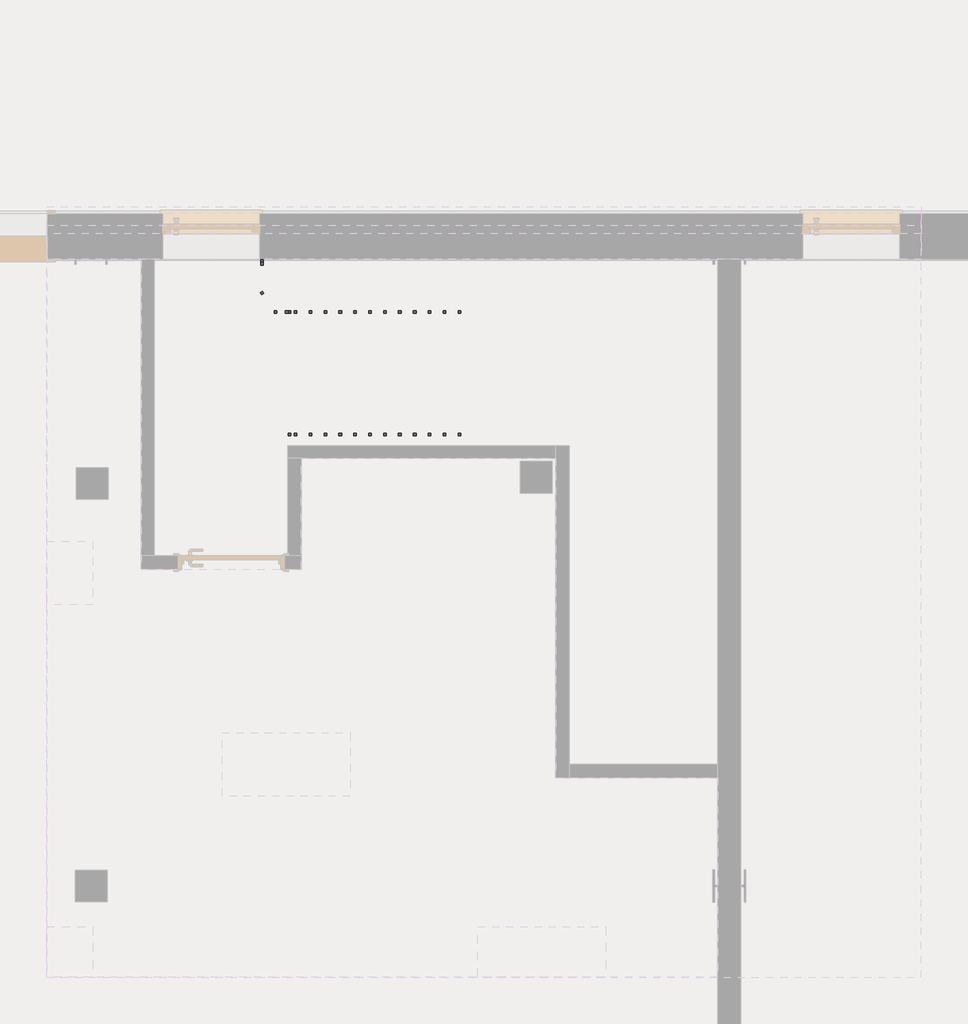
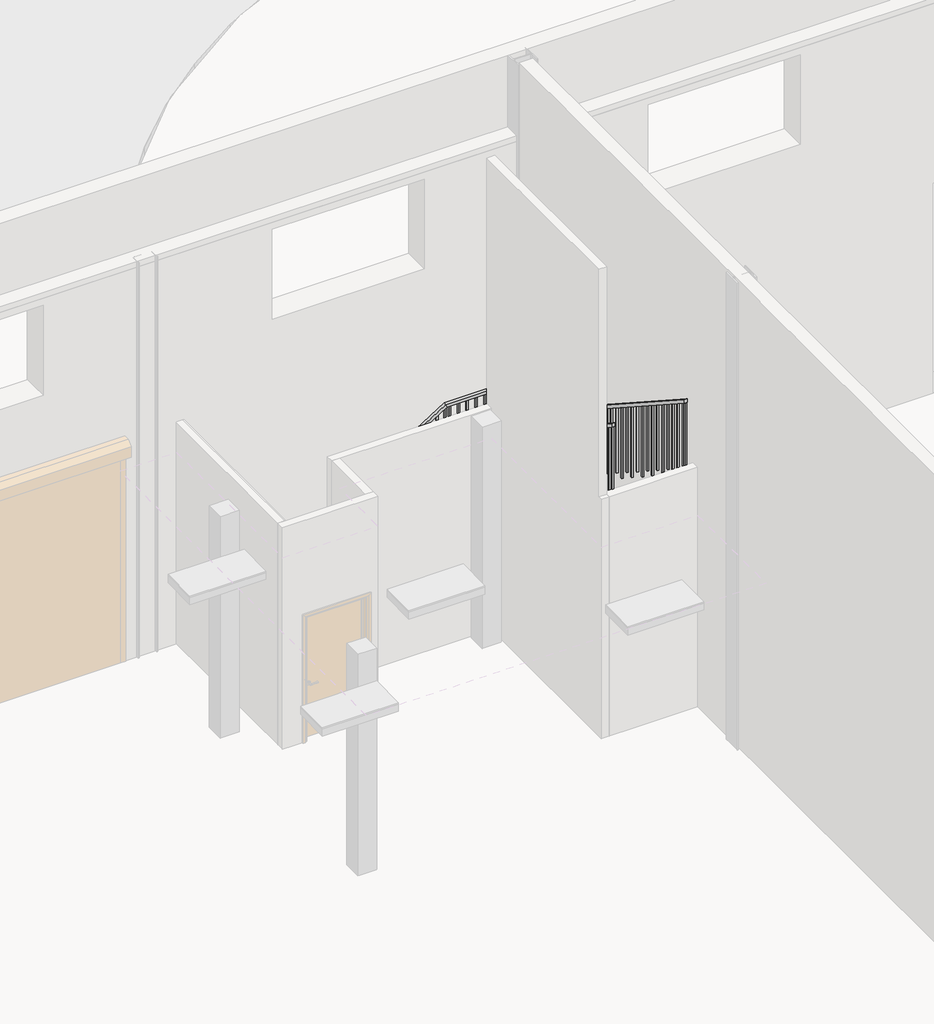
# One storey, part 10 of 13: 3 railings.
"""IFC4 building model written with IfcOpenShell, lengths in millimetres."""

from ifc_helpers import new_model, si_unit, frame, origin, place, context, project, spatial, polyline, outline, extrude, faceted_brep, element, save

model = new_model("IFC4")

# Units and contexts
model_context = context("Model", 3, world=origin())
ifc_project = project(units=[si_unit("LENGTHUNIT", "METRE", prefix="MILLI")], contexts=[model_context])

# Site, building, storey
site = spatial("IfcSite", under=ifc_project)
building = spatial("IfcBuilding", under=site)
storey = spatial("IfcBuildingStorey", under=building, Name="L0 - Ground Floor (Shadows On)", Elevation=0.0)

# Railings
placement = place(None, origin())
element("IfcRailing", 1, ObjectType="1100mm", at=placement, inside=storey, context=model_context, shape_type="SolidModel", body=[
    faceted_brep([(6712.9446543, 5212.4222729, 1286.5612648), (6712.9446543, 5212.4222729, 1227.4016553), (6712.9446543, 5162.4222729, 1227.4016553), (6712.9446543, 5162.4222729, 1286.5612648), (9292.9446543, 5212.4222729, 2918.1818182), (9307.4282868, 5212.4222729, 2868.1818182), (9307.4282868, 5162.4222729, 2868.1818182), (9292.9446543, 5162.4222729, 2918.1818182), (9390.9278057, 5212.4222729, 2918.1818182), (9440.9278057, 5212.4222729, 2868.1818182), (9440.9278057, 5162.4222729, 2868.1818182), (9390.9278057, 5162.4222729, 2918.1818182), (9390.9278057, 5212.4222729, 3148.4415584), (9440.9278057, 5212.4222729, 3098.4415584), (9440.9278057, 5162.4222729, 3098.4415584), (9390.9278057, 5162.4222729, 3148.4415584), (9515.9278057, 5212.4222729, 3148.4415584), (9515.9278057, 5212.4222729, 3098.4415584), (9465.9278057, 5162.4222729, 3098.4415584), (9465.9278057, 5162.4222729, 3148.4415584), (9515.9278057, 5087.4222729, 3148.4415584), (9515.9278057, 5072.6126873, 3098.4415584), (9465.9278057, 5072.6126873, 3098.4415584), (9465.9278057, 5087.4222729, 3148.4415584), (9515.9278057, 2082.0222729, 5100.0), (9465.9278057, 2082.0222729, 5100.0), (9465.9278057, 2082.0222729, 5040.383386), (9515.9278057, 2082.0222729, 5040.383386)], [[[0, 1, 2, 3]], [[1, 0, 4, 5]], [[2, 1, 5, 6]], [[3, 2, 6, 7]], [[0, 3, 7, 4]], [[5, 4, 8, 9]], [[6, 5, 9, 10]], [[7, 6, 10, 11]], [[4, 7, 11, 8]], [[9, 8, 12, 13]], [[10, 9, 13, 14]], [[11, 10, 14, 15]], [[8, 11, 15, 12]], [[13, 12, 16, 17]], [[14, 13, 17, 18]], [[15, 14, 18, 19]], [[12, 15, 19, 16]], [[17, 16, 20, 21]], [[18, 17, 21, 22]], [[19, 18, 22, 23]], [[16, 19, 23, 20]], [[24, 25, 26, 27]], [[21, 20, 24, 27]], [[22, 21, 27, 26]], [[23, 22, 26, 25]], [[20, 23, 25, 24]]]),
    extrude(outline(polyline([(2189.9222729, 4970.3184509), (2189.9222729, 3818.1818182), (2164.9222729, 3818.1818182), (2164.9222729, 4986.5522172), (2189.9222729, 4970.3184509)])), frame((9478.4278057, 0.0, 0.0), z_axis=(1.0, 0.0, 0.0), x_axis=(0.0, 1.0, 0.0)), (0.0, 0.0, 1.0), 25.0),
    extrude(outline(polyline([(2329.9222729, 4879.40936), (2329.9222729, 3818.1818182), (2304.9222729, 3818.1818182), (2304.9222729, 4895.6431263), (2329.9222729, 4879.40936)])), frame((9478.4278057, 0.0, 0.0), z_axis=(1.0, 0.0, 0.0), x_axis=(0.0, 1.0, 0.0)), (0.0, 0.0, 1.0), 25.0),
    extrude(outline(polyline([(2469.9222729, 4788.5002691), (2469.9222729, 3636.3636364), (2444.9222729, 3636.3636364), (2444.9222729, 4804.7340354), (2469.9222729, 4788.5002691)])), frame((9478.4278057, 0.0, 0.0), z_axis=(1.0, 0.0, 0.0), x_axis=(0.0, 1.0, 0.0)), (0.0, 0.0, 1.0), 25.0),
    extrude(outline(polyline([(2609.9222729, 4697.5911782), (2609.9222729, 3636.3636364), (2584.9222729, 3636.3636364), (2584.9222729, 4713.8249444), (2609.9222729, 4697.5911782)])), frame((9478.4278057, 0.0, 0.0), z_axis=(1.0, 0.0, 0.0), x_axis=(0.0, 1.0, 0.0)), (0.0, 0.0, 1.0), 25.0),
    extrude(outline(polyline([(2749.9222729, 4606.6820873), (2749.9222729, 3454.5454545), (2724.9222729, 3454.5454545), (2724.9222729, 4622.9158535), (2749.9222729, 4606.6820873)])), frame((9478.4278057, 0.0, 0.0), z_axis=(1.0, 0.0, 0.0), x_axis=(0.0, 1.0, 0.0)), (0.0, 0.0, 1.0), 25.0),
    extrude(outline(polyline([(2889.9222729, 4515.7729964), (2889.9222729, 3454.5454545), (2864.9222729, 3454.5454545), (2864.9222729, 4532.0067626), (2889.9222729, 4515.7729964)])), frame((9478.4278057, 0.0, 0.0), z_axis=(1.0, 0.0, 0.0), x_axis=(0.0, 1.0, 0.0)), (0.0, 0.0, 1.0), 25.0),
    extrude(outline(polyline([(3029.9222729, 4424.8639055), (3029.9222729, 3272.7272727), (3004.9222729, 3272.7272727), (3004.9222729, 4441.0976717), (3029.9222729, 4424.8639055)])), frame((9478.4278057, 0.0, 0.0), z_axis=(1.0, 0.0, 0.0), x_axis=(0.0, 1.0, 0.0)), (0.0, 0.0, 1.0), 25.0),
    extrude(outline(polyline([(3169.9222729, 4333.9548146), (3169.9222729, 3272.7272727), (3144.9222729, 3272.7272727), (3144.9222729, 4350.1885808), (3169.9222729, 4333.9548146)])), frame((9478.4278057, 0.0, 0.0), z_axis=(1.0, 0.0, 0.0), x_axis=(0.0, 1.0, 0.0)), (0.0, 0.0, 1.0), 25.0),
    extrude(outline(polyline([(3309.9222729, 4243.0457237), (3309.9222729, 3090.9090909), (3284.9222729, 3090.9090909), (3284.9222729, 4259.2794899), (3309.9222729, 4243.0457237)])), frame((9478.4278057, 0.0, 0.0), z_axis=(1.0, 0.0, 0.0), x_axis=(0.0, 1.0, 0.0)), (0.0, 0.0, 1.0), 25.0),
    extrude(outline(polyline([(3449.9222729, 4152.1366328), (3449.9222729, 3090.9090909), (3424.9222729, 3090.9090909), (3424.9222729, 4168.370399), (3449.9222729, 4152.1366328)])), frame((9478.4278057, 0.0, 0.0), z_axis=(1.0, 0.0, 0.0), x_axis=(0.0, 1.0, 0.0)), (0.0, 0.0, 1.0), 25.0),
    extrude(outline(polyline([(3589.9222729, 4061.2275418), (3589.9222729, 2909.0909091), (3564.9222729, 2909.0909091), (3564.9222729, 4077.4613081), (3589.9222729, 4061.2275418)])), frame((9478.4278057, 0.0, 0.0), z_axis=(1.0, 0.0, 0.0), x_axis=(0.0, 1.0, 0.0)), (0.0, 0.0, 1.0), 25.0),
    extrude(outline(polyline([(3729.9222729, 3970.3184509), (3729.9222729, 2909.0909091), (3704.9222729, 2909.0909091), (3704.9222729, 3986.5522172), (3729.9222729, 3970.3184509)])), frame((9478.4278057, 0.0, 0.0), z_axis=(1.0, 0.0, 0.0), x_axis=(0.0, 1.0, 0.0)), (0.0, 0.0, 1.0), 25.0),
    extrude(outline(polyline([(3869.9222729, 3879.40936), (3869.9222729, 2727.2727273), (3844.9222729, 2727.2727273), (3844.9222729, 3895.6431263), (3869.9222729, 3879.40936)])), frame((9478.4278057, 0.0, 0.0), z_axis=(1.0, 0.0, 0.0), x_axis=(0.0, 1.0, 0.0)), (0.0, 0.0, 1.0), 25.0),
    extrude(outline(polyline([(4009.9222729, 3788.5002691), (4009.9222729, 2727.2727273), (3984.9222729, 2727.2727273), (3984.9222729, 3804.7340354), (4009.9222729, 3788.5002691)])), frame((9478.4278057, 0.0, 0.0), z_axis=(1.0, 0.0, 0.0), x_axis=(0.0, 1.0, 0.0)), (0.0, 0.0, 1.0), 25.0),
    extrude(outline(polyline([(4149.9222729, 3697.5911782), (4149.9222729, 2545.4545455), (4124.9222729, 2545.4545455), (4124.9222729, 3713.8249444), (4149.9222729, 3697.5911782)])), frame((9478.4278057, 0.0, 0.0), z_axis=(1.0, 0.0, 0.0), x_axis=(0.0, 1.0, 0.0)), (0.0, 0.0, 1.0), 25.0),
    extrude(outline(polyline([(4289.9222729, 3606.6820873), (4289.9222729, 2545.4545455), (4264.9222729, 2545.4545455), (4264.9222729, 3622.9158535), (4289.9222729, 3606.6820873)])), frame((9478.4278057, 0.0, 0.0), z_axis=(1.0, 0.0, 0.0), x_axis=(0.0, 1.0, 0.0)), (0.0, 0.0, 1.0), 25.0),
    extrude(outline(polyline([(4429.9222729, 3515.7729964), (4429.9222729, 2363.6363636), (4404.9222729, 2363.6363636), (4404.9222729, 3532.0067626), (4429.9222729, 3515.7729964)])), frame((9478.4278057, 0.0, 0.0), z_axis=(1.0, 0.0, 0.0), x_axis=(0.0, 1.0, 0.0)), (0.0, 0.0, 1.0), 25.0),
    extrude(outline(polyline([(4569.9222729, 3424.8639055), (4569.9222729, 2363.6363636), (4544.9222729, 2363.6363636), (4544.9222729, 3441.0976717), (4569.9222729, 3424.8639055)])), frame((9478.4278057, 0.0, 0.0), z_axis=(1.0, 0.0, 0.0), x_axis=(0.0, 1.0, 0.0)), (0.0, 0.0, 1.0), 25.0),
    extrude(outline(polyline([(4709.9222729, 3333.9548146), (4709.9222729, 2181.8181818), (4684.9222729, 2181.8181818), (4684.9222729, 3350.1885808), (4709.9222729, 3333.9548146)])), frame((9478.4278057, 0.0, 0.0), z_axis=(1.0, 0.0, 0.0), x_axis=(0.0, 1.0, 0.0)), (0.0, 0.0, 1.0), 25.0),
    extrude(outline(polyline([(4849.9222729, 3243.0457237), (4849.9222729, 2181.8181818), (4824.9222729, 2181.8181818), (4824.9222729, 3259.2794899), (4849.9222729, 3243.0457237)])), frame((9478.4278057, 0.0, 0.0), z_axis=(1.0, 0.0, 0.0), x_axis=(0.0, 1.0, 0.0)), (0.0, 0.0, 1.0), 25.0),
    extrude(outline(polyline([(4989.9222729, 3152.1366328), (4989.9222729, 2000.0), (4964.9222729, 2000.0), (4964.9222729, 3168.370399), (4989.9222729, 3152.1366328)])), frame((9478.4278057, 0.0, 0.0), z_axis=(1.0, 0.0, 0.0), x_axis=(0.0, 1.0, 0.0)), (0.0, 0.0, 1.0), 25.0),
    extrude(outline(polyline([(9478.4278057, 5129.9222729), (9503.4278057, 5129.9222729), (9503.4278057, 5104.9222729), (9478.4278057, 5104.9222729), (9478.4278057, 5129.9222729)])), frame((0.0, 0.0, 2000.0), z_axis=(0.0, 0.0, 1.0), x_axis=(1.0, 0.0, 0.0)), (0.0, 0.0, 1.0), 1098.4415584),
    extrude(outline(polyline([(9350.4446543, 5174.9222729), (9350.4446543, 5199.9222729), (9375.4446543, 5199.9222729), (9375.4446543, 5174.9222729), (9350.4446543, 5174.9222729)])), frame((0.0, 0.0, 1818.1818182), z_axis=(0.0, 0.0, 1.0), x_axis=(1.0, 0.0, 0.0)), (0.0, 0.0, 1.0), 1050.0),
    extrude(outline(polyline([(2768.9036316, 9150.4446543), (1636.3636364, 9150.4446543), (1636.3636364, 9175.4446543), (2784.7139083, 9175.4446543), (2768.9036316, 9150.4446543)])), frame((0.0, 5174.9222729, 0.0), z_axis=(0.0, 1.0, 0.0), x_axis=(0.0, 0.0, 1.0)), (0.0, 0.0, 1.0), 25.0),
    extrude(outline(polyline([(2680.3660822, 9010.4446543), (1636.3636364, 9010.4446543), (1636.3636364, 9035.4446543), (2696.1763589, 9035.4446543), (2680.3660822, 9010.4446543)])), frame((0.0, 5174.9222729, 0.0), z_axis=(0.0, 1.0, 0.0), x_axis=(0.0, 0.0, 1.0)), (0.0, 0.0, 1.0), 25.0),
    extrude(outline(polyline([(2591.8285328, 8870.4446543), (1454.5454545, 8870.4446543), (1454.5454545, 8895.4446543), (2607.6388095, 8895.4446543), (2591.8285328, 8870.4446543)])), frame((0.0, 5174.9222729, 0.0), z_axis=(0.0, 1.0, 0.0), x_axis=(0.0, 0.0, 1.0)), (0.0, 0.0, 1.0), 25.0),
    extrude(outline(polyline([(2503.2909834, 8730.4446543), (1454.5454545, 8730.4446543), (1454.5454545, 8755.4446543), (2519.1012601, 8755.4446543), (2503.2909834, 8730.4446543)])), frame((0.0, 5174.9222729, 0.0), z_axis=(0.0, 1.0, 0.0), x_axis=(0.0, 0.0, 1.0)), (0.0, 0.0, 1.0), 25.0),
    extrude(outline(polyline([(2414.753434, 8590.4446543), (1272.7272727, 8590.4446543), (1272.7272727, 8615.4446543), (2430.5637107, 8615.4446543), (2414.753434, 8590.4446543)])), frame((0.0, 5174.9222729, 0.0), z_axis=(0.0, 1.0, 0.0), x_axis=(0.0, 0.0, 1.0)), (0.0, 0.0, 1.0), 25.0),
    extrude(outline(polyline([(2326.2158846, 8450.4446543), (1272.7272727, 8450.4446543), (1272.7272727, 8475.4446543), (2342.0261613, 8475.4446543), (2326.2158846, 8450.4446543)])), frame((0.0, 5174.9222729, 0.0), z_axis=(0.0, 1.0, 0.0), x_axis=(0.0, 0.0, 1.0)), (0.0, 0.0, 1.0), 25.0),
    extrude(outline(polyline([(2237.6783352, 8310.4446543), (1090.9090909, 8310.4446543), (1090.9090909, 8335.4446543), (2253.4886119, 8335.4446543), (2237.6783352, 8310.4446543)])), frame((0.0, 5174.9222729, 0.0), z_axis=(0.0, 1.0, 0.0), x_axis=(0.0, 0.0, 1.0)), (0.0, 0.0, 1.0), 25.0),
    extrude(outline(polyline([(2149.1407858, 8170.4446543), (1090.9090909, 8170.4446543), (1090.9090909, 8195.4446543), (2164.9510624, 8195.4446543), (2149.1407858, 8170.4446543)])), frame((0.0, 5174.9222729, 0.0), z_axis=(0.0, 1.0, 0.0), x_axis=(0.0, 0.0, 1.0)), (0.0, 0.0, 1.0), 25.0),
    extrude(outline(polyline([(2060.6032364, 8030.4446543), (909.0909091, 8030.4446543), (909.0909091, 8055.4446543), (2076.413513, 8055.4446543), (2060.6032364, 8030.4446543)])), frame((0.0, 5174.9222729, 0.0), z_axis=(0.0, 1.0, 0.0), x_axis=(0.0, 0.0, 1.0)), (0.0, 0.0, 1.0), 25.0),
    extrude(outline(polyline([(1972.065687, 7890.4446543), (909.0909091, 7890.4446543), (909.0909091, 7915.4446543), (1987.8759636, 7915.4446543), (1972.065687, 7890.4446543)])), frame((0.0, 5174.9222729, 0.0), z_axis=(0.0, 1.0, 0.0), x_axis=(0.0, 0.0, 1.0)), (0.0, 0.0, 1.0), 25.0),
    extrude(outline(polyline([(1883.5281375, 7750.4446543), (727.2727273, 7750.4446543), (727.2727273, 7775.4446543), (1899.3384142, 7775.4446543), (1883.5281375, 7750.4446543)])), frame((0.0, 5174.9222729, 0.0), z_axis=(0.0, 1.0, 0.0), x_axis=(0.0, 0.0, 1.0)), (0.0, 0.0, 1.0), 25.0),
    extrude(outline(polyline([(1794.9905881, 7610.4446543), (727.2727273, 7610.4446543), (727.2727273, 7635.4446543), (1810.8008648, 7635.4446543), (1794.9905881, 7610.4446543)])), frame((0.0, 5174.9222729, 0.0), z_axis=(0.0, 1.0, 0.0), x_axis=(0.0, 0.0, 1.0)), (0.0, 0.0, 1.0), 25.0),
    extrude(outline(polyline([(1706.4530387, 7470.4446543), (545.4545455, 7470.4446543), (545.4545455, 7495.4446543), (1722.2633154, 7495.4446543), (1706.4530387, 7470.4446543)])), frame((0.0, 5174.9222729, 0.0), z_axis=(0.0, 1.0, 0.0), x_axis=(0.0, 0.0, 1.0)), (0.0, 0.0, 1.0), 25.0),
    extrude(outline(polyline([(1617.9154893, 7330.4446543), (545.4545455, 7330.4446543), (545.4545455, 7355.4446543), (1633.725766, 7355.4446543), (1617.9154893, 7330.4446543)])), frame((0.0, 5174.9222729, 0.0), z_axis=(0.0, 1.0, 0.0), x_axis=(0.0, 0.0, 1.0)), (0.0, 0.0, 1.0), 25.0),
    extrude(outline(polyline([(1529.3779399, 7190.4446543), (363.6363636, 7190.4446543), (363.6363636, 7215.4446543), (1545.1882166, 7215.4446543), (1529.3779399, 7190.4446543)])), frame((0.0, 5174.9222729, 0.0), z_axis=(0.0, 1.0, 0.0), x_axis=(0.0, 0.0, 1.0)), (0.0, 0.0, 1.0), 25.0),
    extrude(outline(polyline([(1440.8403905, 7050.4446543), (363.6363636, 7050.4446543), (363.6363636, 7075.4446543), (1456.6506672, 7075.4446543), (1440.8403905, 7050.4446543)])), frame((0.0, 5174.9222729, 0.0), z_axis=(0.0, 1.0, 0.0), x_axis=(0.0, 0.0, 1.0)), (0.0, 0.0, 1.0), 25.0),
    extrude(outline(polyline([(1352.3028411, 6910.4446543), (181.8181818, 6910.4446543), (181.8181818, 6935.4446543), (1368.1131178, 6935.4446543), (1352.3028411, 6910.4446543)])), frame((0.0, 5174.9222729, 0.0), z_axis=(0.0, 1.0, 0.0), x_axis=(0.0, 0.0, 1.0)), (0.0, 0.0, 1.0), 25.0),
    extrude(outline(polyline([(1263.7652917, 6770.4446543), (181.8181818, 6770.4446543), (181.8181818, 6795.4446543), (1279.5755684, 6795.4446543), (1263.7652917, 6770.4446543)])), frame((0.0, 5174.9222729, 0.0), z_axis=(0.0, 1.0, 0.0), x_axis=(0.0, 0.0, 1.0)), (0.0, 0.0, 1.0), 25.0),
    extrude(outline(polyline([(9478.4278057, 5199.9222729), (9503.4278057, 5199.9222729), (9503.4278057, 5174.9222729), (9478.4278057, 5174.9222729), (9478.4278057, 5199.9222729)])), frame((0.0, 0.0, 1818.1818182), z_axis=(0.0, 0.0, 1.0), x_axis=(1.0, 0.0, 0.0)), (0.0, 0.0, 1.0), 1280.2597403),
    extrude(outline(polyline([(2851.1170704, 9280.4446543), (1818.1818182, 9280.4446543), (1818.1818182, 9305.4446543), (2866.927347, 9305.4446543), (2851.1170704, 9280.4446543)])), frame((0.0, 5174.9222729, 0.0), z_axis=(0.0, 1.0, 0.0), x_axis=(0.0, 0.0, 1.0)), (0.0, 0.0, 1.0), 25.0),
    extrude(outline(polyline([(2107.0222729, 5024.1496198), (2107.0222729, 3818.1818182), (2082.0222729, 3818.1818182), (2082.0222729, 5040.383386), (2107.0222729, 5024.1496198)])), frame((9478.4278057, 0.0, 0.0), z_axis=(1.0, 0.0, 0.0), x_axis=(0.0, 1.0, 0.0)), (0.0, 0.0, 1.0), 25.0),
    extrude(outline(polyline([(1227.4016553, 6712.9446543), (181.8181818, 6712.9446543), (181.8181818, 6737.9446543), (1243.211932, 6737.9446543), (1227.4016553, 6712.9446543)])), frame((0.0, 5174.9222729, 0.0), z_axis=(0.0, 1.0, 0.0), x_axis=(0.0, 0.0, 1.0)), (0.0, 0.0, 1.0), 25.0),
])
element("IfcRailing", 2, ObjectType="1100mm", at=placement, inside=storey, context=model_context, shape_type="SolidModel", body=[
    faceted_brep([(6712.9446543, 6361.6222729, 1286.5612648), (6712.9446543, 6361.6222729, 1227.4016553), (6712.9446543, 6311.6222729, 1227.4016553), (6712.9446543, 6311.6222729, 1286.5612648), (9292.9446543, 6361.6222729, 2918.1818182), (9307.4282868, 6361.6222729, 2868.1818182), (9307.4282868, 6311.6222729, 2868.1818182), (9292.9446543, 6311.6222729, 2918.1818182), (10665.1278057, 6361.6222729, 2918.1818182), (10665.1278057, 6361.6222729, 2868.1818182), (10615.1278057, 6311.6222729, 2868.1818182), (10615.1278057, 6311.6222729, 2918.1818182), (10665.1278057, 5442.0222729, 2918.1818182), (10665.1278057, 5427.2126873, 2868.1818182), (10615.1278057, 5427.2126873, 2868.1818182), (10615.1278057, 5442.0222729, 2918.1818182), (10665.1278057, 2082.0222729, 5100.0), (10615.1278057, 2082.0222729, 5100.0), (10615.1278057, 2082.0222729, 5040.383386), (10665.1278057, 2082.0222729, 5040.383386)], [[[0, 1, 2, 3]], [[1, 0, 4, 5]], [[2, 1, 5, 6]], [[3, 2, 6, 7]], [[0, 3, 7, 4]], [[5, 4, 8, 9]], [[6, 5, 9, 10]], [[7, 6, 10, 11]], [[4, 7, 11, 8]], [[9, 8, 12, 13]], [[10, 9, 13, 14]], [[11, 10, 14, 15]], [[8, 11, 15, 12]], [[16, 17, 18, 19]], [[13, 12, 16, 19]], [[14, 13, 19, 18]], [[15, 14, 18, 17]], [[12, 15, 17, 16]]]),
    extrude(outline(polyline([(2164.5222729, 3818.1818182), (2139.5222729, 3818.1818182), (2139.5222729, 5003.0457237), (2164.5222729, 4986.8119574), (2164.5222729, 3818.1818182)])), frame((10627.6278057, 0.0, 0.0), z_axis=(1.0, 0.0, 0.0), x_axis=(0.0, 1.0, 0.0)), (0.0, 0.0, 1.0), 25.0),
    extrude(outline(polyline([(2304.5222729, 3818.1818182), (2279.5222729, 3818.1818182), (2279.5222729, 4912.1366328), (2304.5222729, 4895.9028665), (2304.5222729, 3818.1818182)])), frame((10627.6278057, 0.0, 0.0), z_axis=(1.0, 0.0, 0.0), x_axis=(0.0, 1.0, 0.0)), (0.0, 0.0, 1.0), 25.0),
    extrude(outline(polyline([(2444.5222729, 3636.3636364), (2419.5222729, 3636.3636364), (2419.5222729, 4821.2275418), (2444.5222729, 4804.9937756), (2444.5222729, 3636.3636364)])), frame((10627.6278057, 0.0, 0.0), z_axis=(1.0, 0.0, 0.0), x_axis=(0.0, 1.0, 0.0)), (0.0, 0.0, 1.0), 25.0),
    extrude(outline(polyline([(2584.5222729, 3636.3636364), (2559.5222729, 3636.3636364), (2559.5222729, 4730.3184509), (2584.5222729, 4714.0846847), (2584.5222729, 3636.3636364)])), frame((10627.6278057, 0.0, 0.0), z_axis=(1.0, 0.0, 0.0), x_axis=(0.0, 1.0, 0.0)), (0.0, 0.0, 1.0), 25.0),
    extrude(outline(polyline([(2724.5222729, 3454.5454545), (2699.5222729, 3454.5454545), (2699.5222729, 4639.40936), (2724.5222729, 4623.1755938), (2724.5222729, 3454.5454545)])), frame((10627.6278057, 0.0, 0.0), z_axis=(1.0, 0.0, 0.0), x_axis=(0.0, 1.0, 0.0)), (0.0, 0.0, 1.0), 25.0),
    extrude(outline(polyline([(2864.5222729, 3454.5454545), (2839.5222729, 3454.5454545), (2839.5222729, 4548.5002691), (2864.5222729, 4532.2665029), (2864.5222729, 3454.5454545)])), frame((10627.6278057, 0.0, 0.0), z_axis=(1.0, 0.0, 0.0), x_axis=(0.0, 1.0, 0.0)), (0.0, 0.0, 1.0), 25.0),
    extrude(outline(polyline([(3004.5222729, 3272.7272727), (2979.5222729, 3272.7272727), (2979.5222729, 4457.5911782), (3004.5222729, 4441.357412), (3004.5222729, 3272.7272727)])), frame((10627.6278057, 0.0, 0.0), z_axis=(1.0, 0.0, 0.0), x_axis=(0.0, 1.0, 0.0)), (0.0, 0.0, 1.0), 25.0),
    extrude(outline(polyline([(3144.5222729, 3272.7272727), (3119.5222729, 3272.7272727), (3119.5222729, 4366.6820873), (3144.5222729, 4350.4483211), (3144.5222729, 3272.7272727)])), frame((10627.6278057, 0.0, 0.0), z_axis=(1.0, 0.0, 0.0), x_axis=(0.0, 1.0, 0.0)), (0.0, 0.0, 1.0), 25.0),
    extrude(outline(polyline([(3284.5222729, 3090.9090909), (3259.5222729, 3090.9090909), (3259.5222729, 4275.7729964), (3284.5222729, 4259.5392302), (3284.5222729, 3090.9090909)])), frame((10627.6278057, 0.0, 0.0), z_axis=(1.0, 0.0, 0.0), x_axis=(0.0, 1.0, 0.0)), (0.0, 0.0, 1.0), 25.0),
    extrude(outline(polyline([(3424.5222729, 3090.9090909), (3399.5222729, 3090.9090909), (3399.5222729, 4184.8639055), (3424.5222729, 4168.6301392), (3424.5222729, 3090.9090909)])), frame((10627.6278057, 0.0, 0.0), z_axis=(1.0, 0.0, 0.0), x_axis=(0.0, 1.0, 0.0)), (0.0, 0.0, 1.0), 25.0),
    extrude(outline(polyline([(3564.5222729, 2909.0909091), (3539.5222729, 2909.0909091), (3539.5222729, 4093.9548146), (3564.5222729, 4077.7210483), (3564.5222729, 2909.0909091)])), frame((10627.6278057, 0.0, 0.0), z_axis=(1.0, 0.0, 0.0), x_axis=(0.0, 1.0, 0.0)), (0.0, 0.0, 1.0), 25.0),
    extrude(outline(polyline([(3704.5222729, 2909.0909091), (3679.5222729, 2909.0909091), (3679.5222729, 4003.0457237), (3704.5222729, 3986.8119574), (3704.5222729, 2909.0909091)])), frame((10627.6278057, 0.0, 0.0), z_axis=(1.0, 0.0, 0.0), x_axis=(0.0, 1.0, 0.0)), (0.0, 0.0, 1.0), 25.0),
    extrude(outline(polyline([(3844.5222729, 2727.2727273), (3819.5222729, 2727.2727273), (3819.5222729, 3912.1366328), (3844.5222729, 3895.9028665), (3844.5222729, 2727.2727273)])), frame((10627.6278057, 0.0, 0.0), z_axis=(1.0, 0.0, 0.0), x_axis=(0.0, 1.0, 0.0)), (0.0, 0.0, 1.0), 25.0),
    extrude(outline(polyline([(3984.5222729, 2727.2727273), (3959.5222729, 2727.2727273), (3959.5222729, 3821.2275418), (3984.5222729, 3804.9937756), (3984.5222729, 2727.2727273)])), frame((10627.6278057, 0.0, 0.0), z_axis=(1.0, 0.0, 0.0), x_axis=(0.0, 1.0, 0.0)), (0.0, 0.0, 1.0), 25.0),
    extrude(outline(polyline([(4124.5222729, 2545.4545455), (4099.5222729, 2545.4545455), (4099.5222729, 3730.3184509), (4124.5222729, 3714.0846847), (4124.5222729, 2545.4545455)])), frame((10627.6278057, 0.0, 0.0), z_axis=(1.0, 0.0, 0.0), x_axis=(0.0, 1.0, 0.0)), (0.0, 0.0, 1.0), 25.0),
    extrude(outline(polyline([(4264.5222729, 2545.4545455), (4239.5222729, 2545.4545455), (4239.5222729, 3639.40936), (4264.5222729, 3623.1755938), (4264.5222729, 2545.4545455)])), frame((10627.6278057, 0.0, 0.0), z_axis=(1.0, 0.0, 0.0), x_axis=(0.0, 1.0, 0.0)), (0.0, 0.0, 1.0), 25.0),
    extrude(outline(polyline([(4404.5222729, 2363.6363636), (4379.5222729, 2363.6363636), (4379.5222729, 3548.5002691), (4404.5222729, 3532.2665029), (4404.5222729, 2363.6363636)])), frame((10627.6278057, 0.0, 0.0), z_axis=(1.0, 0.0, 0.0), x_axis=(0.0, 1.0, 0.0)), (0.0, 0.0, 1.0), 25.0),
    extrude(outline(polyline([(4544.5222729, 2363.6363636), (4519.5222729, 2363.6363636), (4519.5222729, 3457.5911782), (4544.5222729, 3441.357412), (4544.5222729, 2363.6363636)])), frame((10627.6278057, 0.0, 0.0), z_axis=(1.0, 0.0, 0.0), x_axis=(0.0, 1.0, 0.0)), (0.0, 0.0, 1.0), 25.0),
    extrude(outline(polyline([(4684.5222729, 2181.8181818), (4659.5222729, 2181.8181818), (4659.5222729, 3366.6820873), (4684.5222729, 3350.4483211), (4684.5222729, 2181.8181818)])), frame((10627.6278057, 0.0, 0.0), z_axis=(1.0, 0.0, 0.0), x_axis=(0.0, 1.0, 0.0)), (0.0, 0.0, 1.0), 25.0),
    extrude(outline(polyline([(4824.5222729, 2181.8181818), (4799.5222729, 2181.8181818), (4799.5222729, 3275.7729964), (4824.5222729, 3259.5392302), (4824.5222729, 2181.8181818)])), frame((10627.6278057, 0.0, 0.0), z_axis=(1.0, 0.0, 0.0), x_axis=(0.0, 1.0, 0.0)), (0.0, 0.0, 1.0), 25.0),
    extrude(outline(polyline([(4964.5222729, 2000.0), (4939.5222729, 2000.0), (4939.5222729, 3184.8639055), (4964.5222729, 3168.6301392), (4964.5222729, 2000.0)])), frame((10627.6278057, 0.0, 0.0), z_axis=(1.0, 0.0, 0.0), x_axis=(0.0, 1.0, 0.0)), (0.0, 0.0, 1.0), 25.0),
    extrude(outline(polyline([(5104.5222729, 2000.0), (5079.5222729, 2000.0), (5079.5222729, 3093.9548146), (5104.5222729, 3077.7210483), (5104.5222729, 2000.0)])), frame((10627.6278057, 0.0, 0.0), z_axis=(1.0, 0.0, 0.0), x_axis=(0.0, 1.0, 0.0)), (0.0, 0.0, 1.0), 25.0),
    extrude(outline(polyline([(5244.5222729, 1818.1818182), (5219.5222729, 1818.1818182), (5219.5222729, 3003.0457237), (5244.5222729, 2986.8119574), (5244.5222729, 1818.1818182)])), frame((10627.6278057, 0.0, 0.0), z_axis=(1.0, 0.0, 0.0), x_axis=(0.0, 1.0, 0.0)), (0.0, 0.0, 1.0), 25.0),
    extrude(outline(polyline([(5384.5222729, 1818.1818182), (5359.5222729, 1818.1818182), (5359.5222729, 2912.1366328), (5384.5222729, 2895.9028665), (5384.5222729, 1818.1818182)])), frame((10627.6278057, 0.0, 0.0), z_axis=(1.0, 0.0, 0.0), x_axis=(0.0, 1.0, 0.0)), (0.0, 0.0, 1.0), 25.0),
    extrude(outline(polyline([(10652.6278057, 5579.1222729), (10652.6278057, 5554.1222729), (10627.6278057, 5554.1222729), (10627.6278057, 5579.1222729), (10652.6278057, 5579.1222729)])), frame((0.0, 0.0, 1818.1818182), z_axis=(0.0, 0.0, 1.0), x_axis=(1.0, 0.0, 0.0)), (0.0, 0.0, 1.0), 1050.0),
    extrude(outline(polyline([(10652.6278057, 5719.1222729), (10652.6278057, 5694.1222729), (10627.6278057, 5694.1222729), (10627.6278057, 5719.1222729), (10652.6278057, 5719.1222729)])), frame((0.0, 0.0, 1818.1818182), z_axis=(0.0, 0.0, 1.0), x_axis=(1.0, 0.0, 0.0)), (0.0, 0.0, 1.0), 1050.0),
    extrude(outline(polyline([(10652.6278057, 5859.1222729), (10652.6278057, 5834.1222729), (10627.6278057, 5834.1222729), (10627.6278057, 5859.1222729), (10652.6278057, 5859.1222729)])), frame((0.0, 0.0, 1818.1818182), z_axis=(0.0, 0.0, 1.0), x_axis=(1.0, 0.0, 0.0)), (0.0, 0.0, 1.0), 1050.0),
    extrude(outline(polyline([(10652.6278057, 5999.1222729), (10652.6278057, 5974.1222729), (10627.6278057, 5974.1222729), (10627.6278057, 5999.1222729), (10652.6278057, 5999.1222729)])), frame((0.0, 0.0, 1818.1818182), z_axis=(0.0, 0.0, 1.0), x_axis=(1.0, 0.0, 0.0)), (0.0, 0.0, 1.0), 1050.0),
    extrude(outline(polyline([(10652.6278057, 6139.1222729), (10652.6278057, 6114.1222729), (10627.6278057, 6114.1222729), (10627.6278057, 6139.1222729), (10652.6278057, 6139.1222729)])), frame((0.0, 0.0, 1818.1818182), z_axis=(0.0, 0.0, 1.0), x_axis=(1.0, 0.0, 0.0)), (0.0, 0.0, 1.0), 1050.0),
    extrude(outline(polyline([(10652.6278057, 6279.1222729), (10652.6278057, 6254.1222729), (10627.6278057, 6254.1222729), (10627.6278057, 6279.1222729), (10652.6278057, 6279.1222729)])), frame((0.0, 0.0, 1818.1818182), z_axis=(0.0, 0.0, 1.0), x_axis=(1.0, 0.0, 0.0)), (0.0, 0.0, 1.0), 1050.0),
    extrude(outline(polyline([(10610.4446543, 6349.1222729), (10635.4446543, 6349.1222729), (10635.4446543, 6324.1222729), (10610.4446543, 6324.1222729), (10610.4446543, 6349.1222729)])), frame((0.0, 0.0, 1818.1818182), z_axis=(0.0, 0.0, 1.0), x_axis=(1.0, 0.0, 0.0)), (0.0, 0.0, 1.0), 1050.0),
    extrude(outline(polyline([(10470.4446543, 6349.1222729), (10495.4446543, 6349.1222729), (10495.4446543, 6324.1222729), (10470.4446543, 6324.1222729), (10470.4446543, 6349.1222729)])), frame((0.0, 0.0, 1818.1818182), z_axis=(0.0, 0.0, 1.0), x_axis=(1.0, 0.0, 0.0)), (0.0, 0.0, 1.0), 1050.0),
    extrude(outline(polyline([(10330.4446543, 6349.1222729), (10355.4446543, 6349.1222729), (10355.4446543, 6324.1222729), (10330.4446543, 6324.1222729), (10330.4446543, 6349.1222729)])), frame((0.0, 0.0, 1818.1818182), z_axis=(0.0, 0.0, 1.0), x_axis=(1.0, 0.0, 0.0)), (0.0, 0.0, 1.0), 1050.0),
    extrude(outline(polyline([(10190.4446543, 6349.1222729), (10215.4446543, 6349.1222729), (10215.4446543, 6324.1222729), (10190.4446543, 6324.1222729), (10190.4446543, 6349.1222729)])), frame((0.0, 0.0, 1818.1818182), z_axis=(0.0, 0.0, 1.0), x_axis=(1.0, 0.0, 0.0)), (0.0, 0.0, 1.0), 1050.0),
    extrude(outline(polyline([(10050.4446543, 6349.1222729), (10075.4446543, 6349.1222729), (10075.4446543, 6324.1222729), (10050.4446543, 6324.1222729), (10050.4446543, 6349.1222729)])), frame((0.0, 0.0, 1818.1818182), z_axis=(0.0, 0.0, 1.0), x_axis=(1.0, 0.0, 0.0)), (0.0, 0.0, 1.0), 1050.0),
    extrude(outline(polyline([(9910.4446543, 6349.1222729), (9935.4446543, 6349.1222729), (9935.4446543, 6324.1222729), (9910.4446543, 6324.1222729), (9910.4446543, 6349.1222729)])), frame((0.0, 0.0, 1818.1818182), z_axis=(0.0, 0.0, 1.0), x_axis=(1.0, 0.0, 0.0)), (0.0, 0.0, 1.0), 1050.0),
    extrude(outline(polyline([(9770.4446543, 6349.1222729), (9795.4446543, 6349.1222729), (9795.4446543, 6324.1222729), (9770.4446543, 6324.1222729), (9770.4446543, 6349.1222729)])), frame((0.0, 0.0, 1818.1818182), z_axis=(0.0, 0.0, 1.0), x_axis=(1.0, 0.0, 0.0)), (0.0, 0.0, 1.0), 1050.0),
    extrude(outline(polyline([(9630.4446543, 6349.1222729), (9655.4446543, 6349.1222729), (9655.4446543, 6324.1222729), (9630.4446543, 6324.1222729), (9630.4446543, 6349.1222729)])), frame((0.0, 0.0, 1818.1818182), z_axis=(0.0, 0.0, 1.0), x_axis=(1.0, 0.0, 0.0)), (0.0, 0.0, 1.0), 1050.0),
    extrude(outline(polyline([(9490.4446543, 6349.1222729), (9515.4446543, 6349.1222729), (9515.4446543, 6324.1222729), (9490.4446543, 6324.1222729), (9490.4446543, 6349.1222729)])), frame((0.0, 0.0, 1818.1818182), z_axis=(0.0, 0.0, 1.0), x_axis=(1.0, 0.0, 0.0)), (0.0, 0.0, 1.0), 1050.0),
    extrude(outline(polyline([(9350.4446543, 6349.1222729), (9375.4446543, 6349.1222729), (9375.4446543, 6324.1222729), (9350.4446543, 6324.1222729), (9350.4446543, 6349.1222729)])), frame((0.0, 0.0, 1818.1818182), z_axis=(0.0, 0.0, 1.0), x_axis=(1.0, 0.0, 0.0)), (0.0, 0.0, 1.0), 1050.0),
    extrude(outline(polyline([(1636.3636364, 9150.4446543), (1636.3636364, 9175.4446543), (2784.7139083, 9175.4446543), (2768.9036316, 9150.4446543), (1636.3636364, 9150.4446543)])), frame((0.0, 6324.1222729, 0.0), z_axis=(0.0, 1.0, 0.0), x_axis=(0.0, 0.0, 1.0)), (0.0, 0.0, 1.0), 25.0),
    extrude(outline(polyline([(1636.3636364, 9010.4446543), (1636.3636364, 9035.4446543), (2696.1763589, 9035.4446543), (2680.3660822, 9010.4446543), (1636.3636364, 9010.4446543)])), frame((0.0, 6324.1222729, 0.0), z_axis=(0.0, 1.0, 0.0), x_axis=(0.0, 0.0, 1.0)), (0.0, 0.0, 1.0), 25.0),
    extrude(outline(polyline([(1454.5454545, 8870.4446543), (1454.5454545, 8895.4446543), (2607.6388095, 8895.4446543), (2591.8285328, 8870.4446543), (1454.5454545, 8870.4446543)])), frame((0.0, 6324.1222729, 0.0), z_axis=(0.0, 1.0, 0.0), x_axis=(0.0, 0.0, 1.0)), (0.0, 0.0, 1.0), 25.0),
    extrude(outline(polyline([(1454.5454545, 8730.4446543), (1454.5454545, 8755.4446543), (2519.1012601, 8755.4446543), (2503.2909834, 8730.4446543), (1454.5454545, 8730.4446543)])), frame((0.0, 6324.1222729, 0.0), z_axis=(0.0, 1.0, 0.0), x_axis=(0.0, 0.0, 1.0)), (0.0, 0.0, 1.0), 25.0),
    extrude(outline(polyline([(1272.7272727, 8590.4446543), (1272.7272727, 8615.4446543), (2430.5637107, 8615.4446543), (2414.753434, 8590.4446543), (1272.7272727, 8590.4446543)])), frame((0.0, 6324.1222729, 0.0), z_axis=(0.0, 1.0, 0.0), x_axis=(0.0, 0.0, 1.0)), (0.0, 0.0, 1.0), 25.0),
    extrude(outline(polyline([(1272.7272727, 8450.4446543), (1272.7272727, 8475.4446543), (2342.0261613, 8475.4446543), (2326.2158846, 8450.4446543), (1272.7272727, 8450.4446543)])), frame((0.0, 6324.1222729, 0.0), z_axis=(0.0, 1.0, 0.0), x_axis=(0.0, 0.0, 1.0)), (0.0, 0.0, 1.0), 25.0),
    extrude(outline(polyline([(1090.9090909, 8310.4446543), (1090.9090909, 8335.4446543), (2253.4886119, 8335.4446543), (2237.6783352, 8310.4446543), (1090.9090909, 8310.4446543)])), frame((0.0, 6324.1222729, 0.0), z_axis=(0.0, 1.0, 0.0), x_axis=(0.0, 0.0, 1.0)), (0.0, 0.0, 1.0), 25.0),
    extrude(outline(polyline([(1090.9090909, 8170.4446543), (1090.9090909, 8195.4446543), (2164.9510624, 8195.4446543), (2149.1407858, 8170.4446543), (1090.9090909, 8170.4446543)])), frame((0.0, 6324.1222729, 0.0), z_axis=(0.0, 1.0, 0.0), x_axis=(0.0, 0.0, 1.0)), (0.0, 0.0, 1.0), 25.0),
    extrude(outline(polyline([(909.0909091, 8030.4446543), (909.0909091, 8055.4446543), (2076.413513, 8055.4446543), (2060.6032364, 8030.4446543), (909.0909091, 8030.4446543)])), frame((0.0, 6324.1222729, 0.0), z_axis=(0.0, 1.0, 0.0), x_axis=(0.0, 0.0, 1.0)), (0.0, 0.0, 1.0), 25.0),
    extrude(outline(polyline([(909.0909091, 7890.4446543), (909.0909091, 7915.4446543), (1987.8759636, 7915.4446543), (1972.065687, 7890.4446543), (909.0909091, 7890.4446543)])), frame((0.0, 6324.1222729, 0.0), z_axis=(0.0, 1.0, 0.0), x_axis=(0.0, 0.0, 1.0)), (0.0, 0.0, 1.0), 25.0),
    extrude(outline(polyline([(727.2727273, 7750.4446543), (727.2727273, 7775.4446543), (1899.3384142, 7775.4446543), (1883.5281375, 7750.4446543), (727.2727273, 7750.4446543)])), frame((0.0, 6324.1222729, 0.0), z_axis=(0.0, 1.0, 0.0), x_axis=(0.0, 0.0, 1.0)), (0.0, 0.0, 1.0), 25.0),
    extrude(outline(polyline([(727.2727273, 7610.4446543), (727.2727273, 7635.4446543), (1810.8008648, 7635.4446543), (1794.9905881, 7610.4446543), (727.2727273, 7610.4446543)])), frame((0.0, 6324.1222729, 0.0), z_axis=(0.0, 1.0, 0.0), x_axis=(0.0, 0.0, 1.0)), (0.0, 0.0, 1.0), 25.0),
    extrude(outline(polyline([(545.4545455, 7470.4446543), (545.4545455, 7495.4446543), (1722.2633154, 7495.4446543), (1706.4530387, 7470.4446543), (545.4545455, 7470.4446543)])), frame((0.0, 6324.1222729, 0.0), z_axis=(0.0, 1.0, 0.0), x_axis=(0.0, 0.0, 1.0)), (0.0, 0.0, 1.0), 25.0),
    extrude(outline(polyline([(545.4545455, 7330.4446543), (545.4545455, 7355.4446543), (1633.725766, 7355.4446543), (1617.9154893, 7330.4446543), (545.4545455, 7330.4446543)])), frame((0.0, 6324.1222729, 0.0), z_axis=(0.0, 1.0, 0.0), x_axis=(0.0, 0.0, 1.0)), (0.0, 0.0, 1.0), 25.0),
    extrude(outline(polyline([(363.6363636, 7190.4446543), (363.6363636, 7215.4446543), (1545.1882166, 7215.4446543), (1529.3779399, 7190.4446543), (363.6363636, 7190.4446543)])), frame((0.0, 6324.1222729, 0.0), z_axis=(0.0, 1.0, 0.0), x_axis=(0.0, 0.0, 1.0)), (0.0, 0.0, 1.0), 25.0),
    extrude(outline(polyline([(363.6363636, 7050.4446543), (363.6363636, 7075.4446543), (1456.6506672, 7075.4446543), (1440.8403905, 7050.4446543), (363.6363636, 7050.4446543)])), frame((0.0, 6324.1222729, 0.0), z_axis=(0.0, 1.0, 0.0), x_axis=(0.0, 0.0, 1.0)), (0.0, 0.0, 1.0), 25.0),
    extrude(outline(polyline([(181.8181818, 6910.4446543), (181.8181818, 6935.4446543), (1368.1131178, 6935.4446543), (1352.3028411, 6910.4446543), (181.8181818, 6910.4446543)])), frame((0.0, 6324.1222729, 0.0), z_axis=(0.0, 1.0, 0.0), x_axis=(0.0, 0.0, 1.0)), (0.0, 0.0, 1.0), 25.0),
    extrude(outline(polyline([(181.8181818, 6770.4446543), (181.8181818, 6795.4446543), (1279.5755684, 6795.4446543), (1263.7652917, 6770.4446543), (181.8181818, 6770.4446543)])), frame((0.0, 6324.1222729, 0.0), z_axis=(0.0, 1.0, 0.0), x_axis=(0.0, 0.0, 1.0)), (0.0, 0.0, 1.0), 25.0),
    extrude(outline(polyline([(10652.6278057, 5454.5222729), (10652.6278057, 5429.5222729), (10627.6278057, 5429.5222729), (10627.6278057, 5454.5222729), (10652.6278057, 5454.5222729)])), frame((0.0, 0.0, 1818.1818182), z_axis=(0.0, 0.0, 1.0), x_axis=(1.0, 0.0, 0.0)), (0.0, 0.0, 1.0), 1050.0),
    extrude(outline(polyline([(10627.6278057, 6349.1222729), (10652.6278057, 6349.1222729), (10652.6278057, 6324.1222729), (10627.6278057, 6324.1222729), (10627.6278057, 6349.1222729)])), frame((0.0, 0.0, 1818.1818182), z_axis=(0.0, 0.0, 1.0), x_axis=(1.0, 0.0, 0.0)), (0.0, 0.0, 1.0), 1050.0),
    extrude(outline(polyline([(1818.1818182, 9280.4446543), (1818.1818182, 9305.4446543), (2866.927347, 9305.4446543), (2851.1170704, 9280.4446543), (1818.1818182, 9280.4446543)])), frame((0.0, 6324.1222729, 0.0), z_axis=(0.0, 1.0, 0.0), x_axis=(0.0, 0.0, 1.0)), (0.0, 0.0, 1.0), 25.0),
    extrude(outline(polyline([(2107.0222729, 3818.1818182), (2082.0222729, 3818.1818182), (2082.0222729, 5040.383386), (2107.0222729, 5024.1496198), (2107.0222729, 3818.1818182)])), frame((10627.6278057, 0.0, 0.0), z_axis=(1.0, 0.0, 0.0), x_axis=(0.0, 1.0, 0.0)), (0.0, 0.0, 1.0), 25.0),
    extrude(outline(polyline([(181.8181818, 6712.9446543), (181.8181818, 6737.9446543), (1243.211932, 6737.9446543), (1227.4016553, 6712.9446543), (181.8181818, 6712.9446543)])), frame((0.0, 6324.1222729, 0.0), z_axis=(0.0, 1.0, 0.0), x_axis=(0.0, 0.0, 1.0)), (0.0, 0.0, 1.0), 25.0),
])
element("IfcRailing", 3, ObjectType="1100mm", at=placement, inside=storey, context=model_context, shape_type="SolidModel", body=[
    faceted_brep([(6712.9446543, 6311.6222729, 1280.0), (6712.9446543, 6311.6222729, 1230.0), (6712.9446543, 6361.6222729, 1230.0), (6712.9446543, 6361.6222729, 1280.0), (6579.9304781, 6311.6222729, 1280.0), (6579.9304781, 6311.6222729, 1230.0), (6605.9588306, 6361.6222729, 1230.0), (6605.9588306, 6361.6222729, 1280.0), (6441.7578383, 6508.9532529, 1280.0), (6441.7578383, 6508.9532529, 1230.0), (6491.7578383, 6524.7181924, 1230.0), (6491.7578383, 6524.7181924, 1280.0), (6441.7578383, 6833.7380918, 1280.0), (6491.7578383, 6833.7380918, 1280.0), (6491.7578383, 6833.7380918, 1230.0), (6441.7578383, 6833.7380918, 1230.0)], [[[0, 1, 2, 3]], [[1, 0, 4, 5]], [[2, 1, 5, 6]], [[3, 2, 6, 7]], [[0, 3, 7, 4]], [[5, 4, 8, 9]], [[6, 5, 9, 10]], [[7, 6, 10, 11]], [[4, 7, 11, 8]], [[12, 13, 14, 15]], [[9, 8, 12, 15]], [[10, 9, 15, 14]], [[11, 10, 14, 13]], [[8, 11, 13, 12]]]),
    extrude(outline(polyline([(6479.2578383, 6779.3357226), (6454.2578383, 6779.3357226), (6454.2578383, 6804.3357226), (6479.2578383, 6804.3357226), (6479.2578383, 6779.3357226)])), frame((0.0, 0.0, 180.0), z_axis=(0.0, 0.0, 1.0), x_axis=(1.0, 0.0, 0.0)), (0.0, 0.0, 1.0), 1050.0),
    extrude(outline(polyline([(6484.1669443, 6513.7660275), (6463.6881432, 6499.4266166), (6449.3487323, 6519.9054177), (6469.8275334, 6534.2448287), (6484.1669443, 6513.7660275)])), frame((0.0, 0.0, 180.0), z_axis=(0.0, 0.0, 1.0), x_axis=(1.0, 0.0, 0.0)), (0.0, 0.0, 1.0), 1050.0),
    extrude(outline(polyline([(6605.4446543, 6349.1222729), (6605.4446543, 6324.1222729), (6580.4446543, 6324.1222729), (6580.4446543, 6349.1222729), (6605.4446543, 6349.1222729)])), frame((0.0, 0.0, 180.0), z_axis=(0.0, 0.0, 1.0), x_axis=(1.0, 0.0, 0.0)), (0.0, 0.0, 1.0), 1050.0),
    extrude(outline(polyline([(6479.2578383, 6808.7380918), (6454.2578383, 6808.7380918), (6454.2578383, 6833.7380918), (6479.2578383, 6833.7380918), (6479.2578383, 6808.7380918)])), frame((0.0, 0.0, 180.0), z_axis=(0.0, 0.0, 1.0), x_axis=(1.0, 0.0, 0.0)), (0.0, 0.0, 1.0), 1050.0),
    extrude(outline(polyline([(6712.9446543, 6349.1222729), (6712.9446543, 6324.1222729), (6687.9446543, 6324.1222729), (6687.9446543, 6349.1222729), (6712.9446543, 6349.1222729)])), frame((0.0, 0.0, 180.0), z_axis=(0.0, 0.0, 1.0), x_axis=(1.0, 0.0, 0.0)), (0.0, 0.0, 1.0), 1050.0),
])

save(model, "model.ifc")

# Revit data of these elements
# Type "1100mm"
#   built-in parameter 1008612 = 0.019685 (stored number, unit not read)
#   built-in parameter 1008611 = 0.019685 (stored number, unit not read)
#   built-in parameter 1008609 = 0.902231 (stored number, unit not read)
#   built-in parameter 1008604 = 0.19685 (stored number, unit not read)
#   built-in parameter 1008603 = 0.164042 (stored number, unit not read)
#   Railing Height = 1100 mm
#   built-in parameter 1008630 = 2
#   built-in parameter 1008610 = 2
#   built-in parameter 1008608 = 1
#   built-in parameter 1008618 = Baluster - Square : 25mm
# Elements 1, 2 (IfcRailing, "1100mm")
#   Phase Created = New Construction
# Element 3 (IfcRailing, "1100mm")
#   built-in parameter 1008621 = 0.590551 (stored number, unit not read)
#   Phase Created = New Construction
